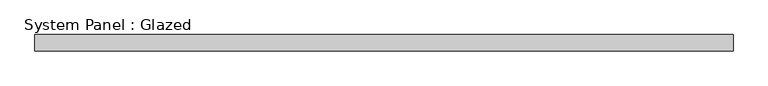
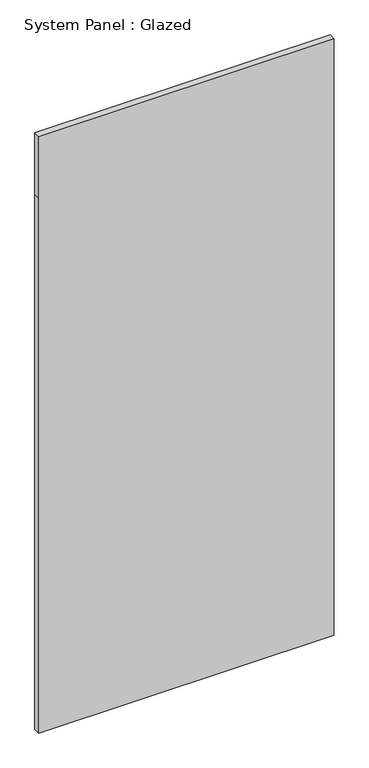
"""IFC4 building model written with IfcOpenShell, lengths in millimetres: plate geometry, System Panel : Glazed."""

from ifc_helpers import new_model, si_unit, frame, origin, place, context, project, spatial, polyline, outline, extrude, source, transform, mapped, element, save


def system_panel_glazed_1fc46e14(model_context):
    return source(origin(), model_context, "Body", "SweptSolid", [
        extrude(outline(polyline([(0.0, -549.275), (0.0, 549.275), (2101.85, 549.275), (2343.15, 549.275), (2343.15, -549.275), (2101.85, -549.275), (0.0, -549.275)])), frame((0.0, 19.05, 0.0), z_axis=(0.0, 1.0, 0.0), x_axis=(0.0, 0.0, 1.0)), (0.0, 0.0, 1.0), 25.4),
    ])


if __name__ == "__main__":
    model = new_model("IFC4")
    model_context = context("Model", 3, world=origin())
    ifc_project = project(units=[si_unit("LENGTHUNIT", "METRE", prefix="MILLI")], contexts=[model_context])
    site = spatial("IfcSite", under=ifc_project)
    building = spatial("IfcBuilding", under=site)
    placement = place(None, origin())
    system_panel_glazed_shape = system_panel_glazed_1fc46e14(model_context)
    element("IfcPlate", 1, ObjectType="System Panel : Glazed", at=placement, inside=building, context=model_context, shape_type="MappedRepresentation", body=[
        mapped(system_panel_glazed_shape, transform((0.0, 0.0, 0.0), x_axis=(1.0, 0.0, 0.0), y_axis=(0.0, 1.0, 0.0), z_axis=(0.0, 0.0, 1.0))),
    ])
    save(model, "model.ifc")

# Revit data of these elements
# Element 1 (IfcPlate, "System Panel : Glazed")
#   Materials on its faces: "Glass"
# Materials
#   "Glass": class "Glass", colour RGB 0 128 192, transparency 0.75
